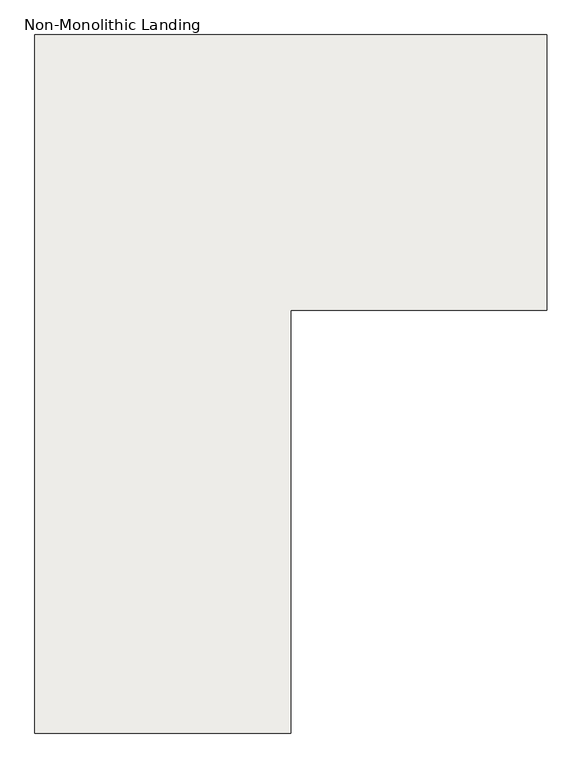
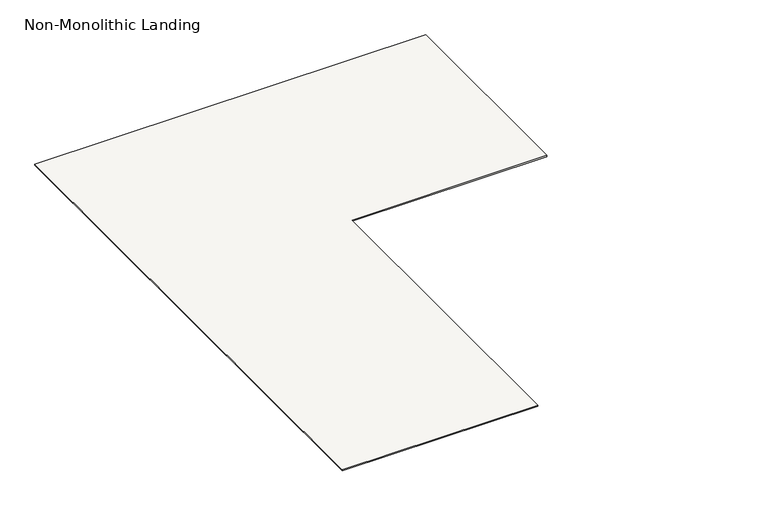
"""IFC4 building model written with IfcOpenShell, lengths in millimetres: slab geometry, Non-Monolithic Landing."""

from ifc_helpers import new_model, si_unit, origin, place, context, project, spatial, faceted_brep, source, transform, mapped, element, save


def non_monolithic_landing_c36497a5(model_context):
    return source(origin(), model_context, "Body", "Brep", [
        faceted_brep([(14425.0, 13214.4345331, 32000.0), (12225.0, 13214.4345331, 32000.0), (12225.0, 10214.4345331, 32000.0), (13325.0, 10214.4345331, 32000.0), (13325.0, 12030.4345331, 32000.0), (14425.0, 12030.4345331, 32000.0), (12225.0, 10214.4345331, 31994.0), (12225.0, 13214.4345331, 31994.0), (14424.15, 13214.4345331, 31994.0), (14424.15, 12030.4345331, 31994.0), (13325.0, 12030.4345331, 31994.0), (13325.0, 10214.4345331, 31994.0)], [[[0, 1, 2, 3, 4, 5]], [[6, 7, 8, 9, 10, 11]], [[1, 0, 8, 7]], [[5, 4, 10, 9]], [[4, 3, 11, 10]], [[3, 2, 6, 11]], [[2, 1, 7, 6]], [[0, 5, 9, 8]]]),
    ])


if __name__ == "__main__":
    model = new_model("IFC4")
    model_context = context("Model", 3, world=origin())
    ifc_project = project(units=[si_unit("LENGTHUNIT", "METRE", prefix="MILLI")], contexts=[model_context])
    site = spatial("IfcSite", under=ifc_project)
    building = spatial("IfcBuilding", under=site)
    placement = place(None, origin())
    non_monolithic_landing_shape = non_monolithic_landing_c36497a5(model_context)
    element("IfcSlab", 1, ObjectType="Non-Monolithic Landing", at=placement, inside=building, context=model_context, shape_type="MappedRepresentation", body=[
        mapped(non_monolithic_landing_shape, transform((0.0, 0.0, 0.0), x_axis=(1.0, 0.0, 0.0), y_axis=(0.0, 1.0, 0.0), z_axis=(0.0, 0.0, 1.0))),
    ])
    save(model, "model.ifc")

# Revit data of these elements
# Element 1 (IfcSlab, "Non-Monolithic Landing")
#   Materials on its faces: "Steel, Paint Finish, Dark Gray"
# Materials
#   "Steel, Paint Finish, Dark Gray": class "Metal", colour RGB 89 89 89, transparency 0, Description = "Steel, paint finish, dark gray, glossy", Cost = 0
